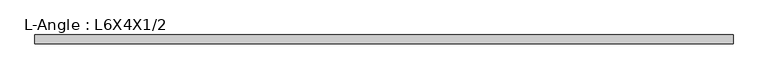
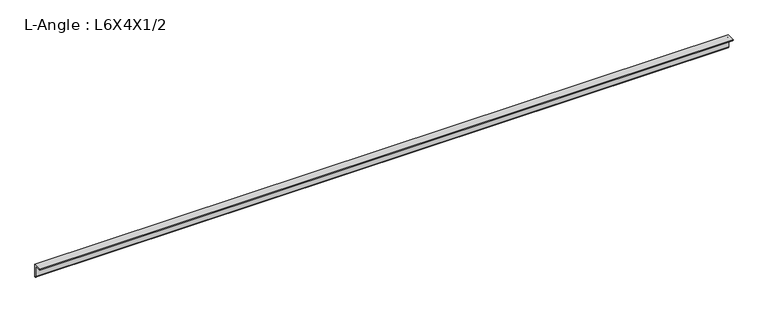
"""IFC4 building model written with IfcOpenShell, lengths in millimetres: beam geometry, L-Angle : L6X4X1/2."""

from ifc_helpers import new_model, si_unit, point, frame, frame_2d, origin, place, context, project, spatial, polyline, circle_curve, trimmed, segment, composite_curve, outline, extrude, source, transform, mapped, element, save


def l_angle_l6x4x1_2_20ef610f(model_context):
    return source(origin(), model_context, "Body", "SweptSolid", [
        extrude(outline(composite_curve([segment(polyline([(24.9174, 50.292), (24.9174, -102.108)]), True, "CONTINUOUS"), segment(trimmed(circle_curve(frame_2d((24.9174, -89.408)), 12.7), [point((24.9174, -102.108))], [point((12.2174, -89.408))], False, "CARTESIAN"), True, "CONTINUOUS"), segment(polyline([(12.2174, -89.408), (12.2174, 24.892)]), True, "CONTINUOUS"), segment(trimmed(circle_curve(frame_2d((-0.4826, 24.892)), 12.7), [point((12.2174, 24.892))], [point((-0.4826, 37.592))], True, "CARTESIAN"), True, "CONTINUOUS"), segment(polyline([(-0.4826, 37.592), (-63.9826, 37.592)]), True, "CONTINUOUS"), segment(trimmed(circle_curve(frame_2d((-63.9826, 50.292)), 12.7), [point((-63.9826, 37.592))], [point((-76.6826, 50.292))], False, "CARTESIAN"), True, "CONTINUOUS"), segment(polyline([(-76.6826, 50.292), (24.9174, 50.292)]), True, "CONTINUOUS")], self_intersect=False)), frame((-4009.4734549, 0.0, 0.0), z_axis=(1.0, 0.0, 0.0), x_axis=(0.0, 1.0, 0.0)), (0.0, 0.0, 1.0), 7993.1205549),
    ])


if __name__ == "__main__":
    model = new_model("IFC4")
    model_context = context("Model", 3, world=origin())
    ifc_project = project(units=[si_unit("LENGTHUNIT", "METRE", prefix="MILLI")], contexts=[model_context])
    site = spatial("IfcSite", under=ifc_project)
    building = spatial("IfcBuilding", under=site)
    placement = place(None, origin())
    l_angle_l6x4x1_2_shape = l_angle_l6x4x1_2_20ef610f(model_context)
    element("IfcBeam", 1, ObjectType="L-Angle : L6X4X1/2", at=placement, inside=building, context=model_context, shape_type="MappedRepresentation", body=[
        mapped(l_angle_l6x4x1_2_shape, transform((0.0, 0.0, 0.0), x_axis=(1.0, 0.0, 0.0), y_axis=(0.0, 1.0, 0.0), z_axis=(0.0, 0.0, 1.0))),
    ])
    save(model, "model.ifc")

# Revit data of these elements
# Type "L-Angle : L6X4X1/2"
#   Assembly Code = "B10"
#   k = 0' - 1"
#   W = 16.2
#   Length [instance default] = 5' - 0"
#   b = 0' - 4"
#   d = 0' - 6"
#   t = 0' - 0 1/2"
#   x = 0' - 0.981"
#   y = 0' - 1.98"
#   A = 0.0329861 SF
#   Structural Material [instance default] = Steel ASTM A36
# Element 1 (IfcBeam, "L-Angle : L6X4X1/2")
#   Materials on its faces: "Steel ASTM A36"
# Materials
#   "Steel ASTM A36": class "Metal", colour RGB 199 199 199, transparency 0, Description = "Structural steel, ASTM A36 Grade B, mill finish", Cost = 0
